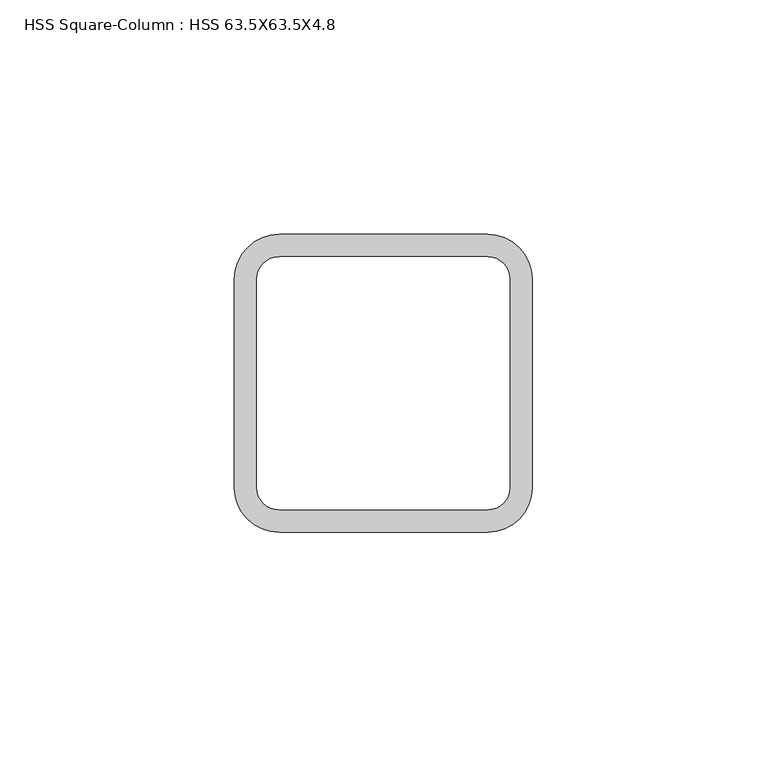
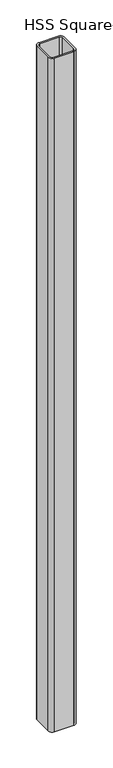
"""IFC4 building model written with IfcOpenShell, lengths in millimetres: column geometry, HSS Square-Column : HSS 63.5X63.5X4.8."""

from ifc_helpers import new_model, si_unit, point, frame, frame_2d, origin, place, context, project, spatial, polyline, circle_curve, trimmed, segment, composite_curve, outline, extrude, source, transform, mapped, element, save


def hss_square_column_hss_63_5x63_5x4_8_5112d7a3(model_context):
    return source(origin(), model_context, "Body", "SweptSolid", [
        extrude(outline(composite_curve([segment(trimmed(circle_curve(frame_2d((22.225, 22.225)), 9.525), [point((22.225, 31.75))], [point((31.75, 22.225))], False, "CARTESIAN"), True, "CONTINUOUS"), segment(polyline([(31.75, 22.225), (31.75, -22.225)]), True, "CONTINUOUS"), segment(trimmed(circle_curve(frame_2d((22.225, -22.225)), 9.525), [point((31.75, -22.225))], [point((22.225, -31.75))], False, "CARTESIAN"), True, "CONTINUOUS"), segment(polyline([(22.225, -31.75), (-22.225, -31.75)]), True, "CONTINUOUS"), segment(trimmed(circle_curve(frame_2d((-22.225, -22.225)), 9.525), [point((-22.225, -31.75))], [point((-31.75, -22.225))], False, "CARTESIAN"), True, "CONTINUOUS"), segment(polyline([(-31.75, -22.225), (-31.75, 22.225)]), True, "CONTINUOUS"), segment(trimmed(circle_curve(frame_2d((-22.225, 22.225)), 9.525), [point((-31.75, 22.225))], [point((-22.225, 31.75))], False, "CARTESIAN"), True, "CONTINUOUS"), segment(polyline([(-22.225, 31.75), (22.225, 31.75)]), True, "CONTINUOUS")], self_intersect=False), holes=[composite_curve([segment(polyline([(22.225, 26.9875), (-22.225, 26.9875)]), True, "CONTINUOUS"), segment(trimmed(circle_curve(frame_2d((-22.225, 22.225)), 4.7625), [point((-22.225, 26.9875))], [point((-26.9875, 22.225))], True, "CARTESIAN"), True, "CONTINUOUS"), segment(polyline([(-26.9875, 22.225), (-26.9875, -22.225)]), True, "CONTINUOUS"), segment(trimmed(circle_curve(frame_2d((-22.225, -22.225)), 4.7625), [point((-26.9875, -22.225))], [point((-22.225, -26.9875))], True, "CARTESIAN"), True, "CONTINUOUS"), segment(polyline([(-22.225, -26.9875), (22.225, -26.9875)]), True, "CONTINUOUS"), segment(trimmed(circle_curve(frame_2d((22.225, -22.225)), 4.7625), [point((22.225, -26.9875))], [point((26.9875, -22.225))], True, "CARTESIAN"), True, "CONTINUOUS"), segment(polyline([(26.9875, -22.225), (26.9875, 22.225)]), True, "CONTINUOUS"), segment(trimmed(circle_curve(frame_2d((22.225, 22.225)), 4.7625), [point((26.9875, 22.225))], [point((22.225, 26.9875))], True, "CARTESIAN"), True, "CONTINUOUS")], self_intersect=False)]), frame((0.0, 0.0, 3220.0), z_axis=(0.0, 0.0, 1.0), x_axis=(1.0, 0.0, 0.0)), (0.0, 0.0, 1.0), 1650.0),
    ])


if __name__ == "__main__":
    model = new_model("IFC4")
    model_context = context("Model", 3, world=origin())
    ifc_project = project(units=[si_unit("LENGTHUNIT", "METRE", prefix="MILLI")], contexts=[model_context])
    site = spatial("IfcSite", under=ifc_project)
    building = spatial("IfcBuilding", under=site)
    placement = place(None, origin())
    hss_square_column_hss_63_5x63_5x4_8_shape = hss_square_column_hss_63_5x63_5x4_8_5112d7a3(model_context)
    element("IfcColumn", 1, ObjectType="HSS Square-Column : HSS 63.5X63.5X4.8", at=placement, inside=building, context=model_context, shape_type="MappedRepresentation", body=[
        mapped(hss_square_column_hss_63_5x63_5x4_8_shape, transform((0.0, 0.0, 0.0), x_axis=(1.0, 0.0, 0.0), y_axis=(0.0, 1.0, 0.0), z_axis=(0.0, 0.0, 1.0))),
    ])
    save(model, "model.ifc")

# Revit data of these elements
# Type "HSS Square-Column : HSS 63.5X63.5X4.8"
#   Section Name Key = "HSS 2 1/2X2 1/2X3/16"
#   Assembly Code = "B10"
#   Width = 6.35 cm
#   Wall Nominal Thickness = 0.4763 cm
#   Wall Design Thickness = 0.442 cm
#   Torsional Moment of Inertia = 93.6521 cm⁴
#   Torsional Modulus = 30.4799 cm³
#   Section Area = 9.93546 cm²
#   Plastic Modulus weak axis = 21.6309 cm³
#   Plastic Modulus strong axis = 21.6309 cm³
#   Outer Fillet = 0.9525 cm
#   Nominal Weight = 8.31884 kgf/m
#   Moment of Inertia weak axis = 56.1912 cm⁴
#   Moment of Inertia strong axis = 56.1912 cm⁴
#   Inner Fillet = 0.4763 cm
#   Height = 6.35 cm
#   Elastic Modulus weak axis = 17.698 cm³
#   Elastic Modulus strong axis = 17.698 cm³
#   Centroid Vertical = 3.175 cm
#   Centroid Horizontal = 3.175 cm
#   Structural Material [instance default] = Steel ASTM A500, Grade B, Rectangular and Square
#   Principal Axes Angle = 0
# Element 1 (IfcColumn, "HSS Square-Column : HSS 63.5X63.5X4.8")
#   Structural Material = none
# Materials
#   "Steel ASTM A500, Grade B, Rectangular and Square": class "Metal", colour RGB 199 199 199, transparency 0, Description = "Carbon steel", Cost = 0
